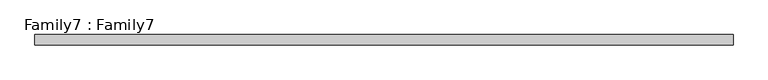
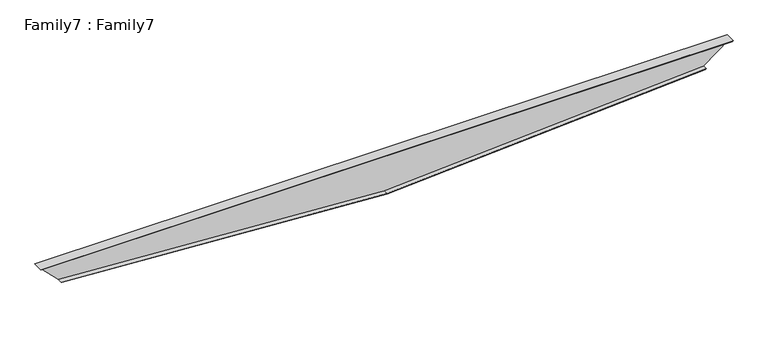
"""IFC4 building model written with IfcOpenShell, lengths in millimetres: beam geometry, Family7 : Family7."""

from ifc_helpers import new_model, si_unit, frame, origin, place, context, project, spatial, polyline, outline, extrude, source, transform, mapped, element, save


def family7_family7_14774666(model_context):
    return source(origin(), model_context, "Body", "SweptSolid", [
        extrude(outline(polyline([(-914.4, -14659.3825135), (-1828.8, 0.0), (-914.4, 14336.786696), (-31.75, 15508.1028078), (-31.75, -15542.0325135), (-914.4, -14659.3825135)])), frame((0.0, -15.875, 0.0), z_axis=(0.0, 1.0, 0.0), x_axis=(0.0, 0.0, 1.0)), (0.0, 0.0, 1.0), 31.75),
        extrude(outline(polyline([(-914.4, 14336.786696), (-1828.8, 0.0), (-914.4, -14659.3825135), (-948.3280154, -14625.4544981), (-1860.6130939, 0.0222371), (-949.1562421, 14290.6636049), (-914.4, 14336.786696)])), frame((0.0, -228.6, 0.0), z_axis=(0.0, 1.0, 0.0), x_axis=(0.0, 0.0, 1.0)), (0.0, 0.0, 1.0), 457.2),
        extrude(outline(polyline([(-31.75, 15508.1028078), (0.0, 15550.2364809), (0.0, -15573.7825135), (-31.75, -15542.0325135), (-31.75, 15508.1028078)])), frame((0.0, -228.6, 0.0), z_axis=(0.0, 1.0, 0.0), x_axis=(0.0, 0.0, 1.0)), (0.0, 0.0, 1.0), 457.2),
    ])


if __name__ == "__main__":
    model = new_model("IFC4")
    model_context = context("Model", 3, world=origin())
    ifc_project = project(units=[si_unit("LENGTHUNIT", "METRE", prefix="MILLI")], contexts=[model_context])
    site = spatial("IfcSite", under=ifc_project)
    building = spatial("IfcBuilding", under=site)
    placement = place(None, origin())
    family7_family7_shape = family7_family7_14774666(model_context)
    element("IfcBeam", 1, ObjectType="Family7 : Family7", at=placement, inside=building, context=model_context, shape_type="MappedRepresentation", body=[
        mapped(family7_family7_shape, transform((0.0, 0.0, 0.0), x_axis=(1.0, 0.0, 0.0), y_axis=(0.0, 1.0, 0.0), z_axis=(0.0, 0.0, 1.0))),
    ])
    save(model, "model.ifc")

# Revit data of these elements
# Type "Family7 : Family7"
#   Width = 1' - 6"
#   Web_Thickness = 0' - 1 1/4"
#   Length [instance default] = 69' - 10"
#   Depth_Mid [instance default] = 6' - 0"
#   Depth_End = 3' - 0"
#   Angle_Right = 53.00°
#   Angle_Left = 45.00°
